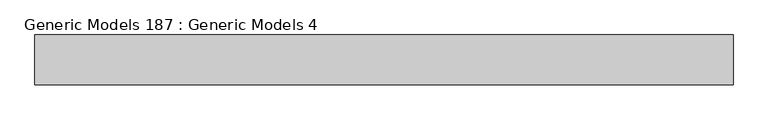
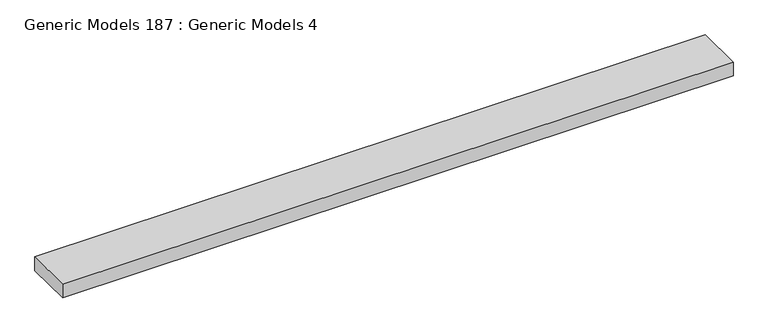
"""IFC4 building model written with IfcOpenShell, lengths in millimetres: proxy geometry, Generic Models 187 : Generic Models 4."""

from ifc_helpers import new_model, si_unit, frame, origin, place, context, project, spatial, polyline, outline, extrude, source, transform, mapped, element, save


def generic_models_187_generic_models_4_d8c55f5b(model_context):
    return source(origin(), model_context, "Body", "SweptSolid", [
        extrude(outline(polyline([(2196.9263704, -4512.1424801), (2196.9263704, -5400.9181208), (-10256.7421316, -5400.9181208), (-10256.7421316, -4512.1424801), (2196.9263704, -4512.1424801)])), frame((0.0, 0.0, 126489.9460277), z_axis=(0.0, 0.0, 1.0), x_axis=(1.0, 0.0, 0.0)), (0.0, 0.0, 1.0), 266.7),
    ])


if __name__ == "__main__":
    model = new_model("IFC4")
    model_context = context("Model", 3, world=origin())
    ifc_project = project(units=[si_unit("LENGTHUNIT", "METRE", prefix="MILLI")], contexts=[model_context])
    site = spatial("IfcSite", under=ifc_project)
    building = spatial("IfcBuilding", under=site)
    placement = place(None, origin())
    generic_models_187_generic_models_4_shape = generic_models_187_generic_models_4_d8c55f5b(model_context)
    element("IfcBuildingElementProxy", 1, Name="Generic Models 187 : Generic Models 4", ObjectType="Generic Models 187 : Generic Models 4", at=placement, inside=building, context=model_context, shape_type="MappedRepresentation", body=[
        mapped(generic_models_187_generic_models_4_shape, transform((0.0, 0.0, 0.0), x_axis=(1.0, 0.0, 0.0), y_axis=(0.0, 1.0, 0.0), z_axis=(0.0, 0.0, 1.0))),
    ])
    save(model, "model.ifc")

# Revit data of these elements
# Element 1 (IfcBuildingElementProxy, "Generic Models 187 : Generic Models 4")
#   Materials on its faces: "_SOUND BATT INSULATION"
# Materials
#   "_SOUND BATT INSULATION": class "Generic", colour RGB 245 226 173, transparency 0, Cost = 0
